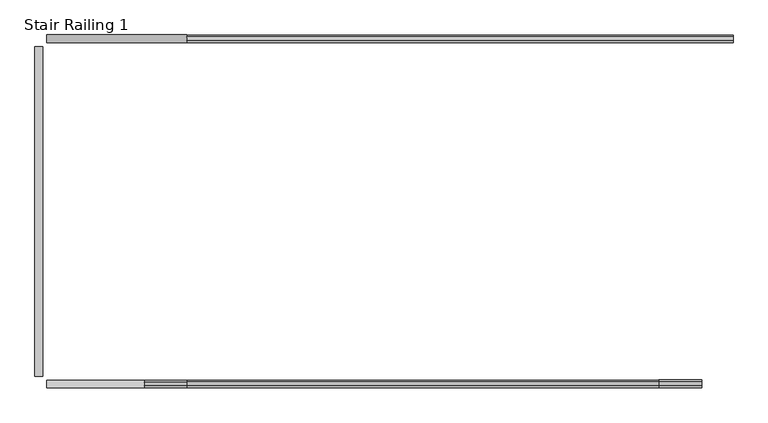
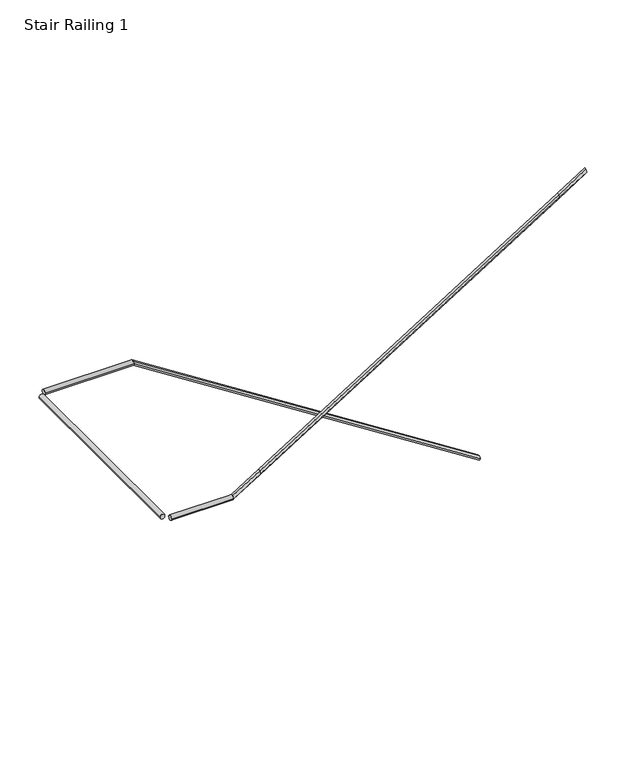
"""IFC4 building model written with IfcOpenShell, lengths in millimetres: railing geometry, Stair Railing 1."""

import ifcopenshell
import ifcopenshell.guid

model = None  # the IFC model being written
_history = None  # IfcOwnerHistory: only IFC2X3 demands one
_inside = {}  # id of a spatial element -> (the spatial element, [elements in it])
_under = {}  # id of a project, library or spatial element -> (it, [spatial elements below it])
_declared = {}  # id of a project -> (the project, [libraries it declares])
_typed = {}  # id of a type object -> (the type object, [elements of that type])
_made_of = {}  # id of a material, layer set ... -> (it, [elements and type objects made of it])


def new_model(schema):
    """Start an empty IFC model of exactly this schema.

    Asked for "IFC4X3", IfcOpenShell would pick the latest addendum, in which some entities
    have other attributes; the version numbers below select the first issue.
    IFC2X3 requires an IfcOwnerHistory on every rooted entity: one is made here for all.
    """
    global model, _history
    if schema == "IFC4X3":
        model = ifcopenshell.file(schema_version=(4, 3, 0, 0))
    else:
        model = ifcopenshell.file(schema=schema)
    _inside.clear()
    _under.clear()
    _declared.clear()
    _typed.clear()
    _made_of.clear()
    _history = None
    if model.schema == "IFC2X3":
        org = make("IfcOrganization", Name="unknown")
        user = make(
            "IfcPersonAndOrganization",
            ThePerson=make("IfcPerson", FamilyName="unknown"),
            TheOrganization=org,
        )
        app = make(
            "IfcApplication",
            ApplicationDeveloper=org,
            Version="unknown",
            ApplicationFullName="unknown",
            ApplicationIdentifier="unknown",
        )
        _history = make(
            "IfcOwnerHistory",
            OwningUser=user,
            OwningApplication=app,
            ChangeAction="ADDED",
            CreationDate=0,
        )
    return model


def make(cls, **values):
    """One entity of the class cls with the attributes given. An attribute that is None is left unset."""
    return model.create_entity(
        cls, **{name: value for name, value in values.items() if value is not None}
    )


def rooted(cls, **values):
    """An entity with a GlobalId (a new one), such as an element, a storey or a relation."""
    return make(cls, GlobalId=ifcopenshell.guid.new(), OwnerHistory=_history, **values)


def si_unit(unit_type, name, prefix=None):
    """IfcSIUnit, for example si_unit("LENGTHUNIT", "METRE", prefix="MILLI")."""
    return make("IfcSIUnit", UnitType=unit_type, Prefix=prefix, Name=name)


def assignment(units):
    """IfcUnitAssignment: the units of a project."""
    return None if units is None else make("IfcUnitAssignment", Units=units)


def point(xyz):
    """IfcCartesianPoint."""
    return None if xyz is None else make("IfcCartesianPoint", Coordinates=xyz)


def direction(xyz):
    """IfcDirection."""
    return None if xyz is None else make("IfcDirection", DirectionRatios=xyz)


def frame(location, z_axis=None, x_axis=None):
    """IfcAxis2Placement3D, a coordinate frame: its origin and axes. An axis left out is left unset."""
    return make(
        "IfcAxis2Placement3D",
        Location=point(location),
        Axis=direction(z_axis),
        RefDirection=direction(x_axis),
    )


def origin():
    """The frame at (0, 0, 0) with its axes left unset."""
    return frame((0.0, 0.0, 0.0))


def place(relative_to, where):
    """IfcLocalPlacement: puts the frame where relative to a parent placement (None: the world)."""
    return make(
        "IfcLocalPlacement", PlacementRelTo=relative_to, RelativePlacement=where
    )


def context(
    kind, dimensions, precision=None, world=None, true_north=None, identifier=None
):
    """IfcGeometricRepresentationContext, for example the 3D "Model" context."""
    return make(
        "IfcGeometricRepresentationContext",
        ContextIdentifier=identifier,
        ContextType=kind,
        CoordinateSpaceDimension=dimensions,
        Precision=precision,
        WorldCoordinateSystem=world,
        TrueNorth=true_north,
    )


def project(units=None, contexts=None):
    """IfcProject with its units and contexts."""
    return rooted(
        "IfcProject",
        Name="project",
        RepresentationContexts=contexts,
        UnitsInContext=assignment(units),
    )


def spatial(cls, under=None, at=None, **own):
    """A site, building, storey or space (cls), placed at a placement, below another one or the project."""
    s = rooted(cls, ObjectPlacement=at, **own)
    if under is not None:
        _under.setdefault(under.id(), (under, []))[1].append(s)
    return s


def circle_curve(where, radius):
    """IfcCircle in the frame where."""
    return make("IfcCircle", Position=where, Radius=radius)


def faces_of(points, faces, orient=None, outer=None):
    """IfcFace entities. A face is a list of loops; a loop is a list of indices into points, from 0.

    orient and outer hold one flag for each loop. By default every Orientation is true, the
    first loop of a face is its IfcFaceOuterBound and the others are IfcFaceBound.
    """
    made = []
    for i, loops in enumerate(faces):
        bounds = []
        for j, loop in enumerate(loops):
            is_outer = j == 0 if outer is None else outer[i][j]
            bounds.append(
                make(
                    "IfcFaceOuterBound" if is_outer else "IfcFaceBound",
                    Bound=make("IfcPolyLoop", Polygon=[points[k] for k in loop]),
                    Orientation=True if orient is None else orient[i][j],
                )
            )
        made.append(make("IfcFace", Bounds=bounds))
    return made


def faceted_brep(points, faces, orient=None, outer=None, voids=None):
    """IfcFacetedBrep: a solid bounded by flat faces; with voids (closed shells), ...WithVoids."""
    shared = [point(p) for p in points]
    hull = make("IfcClosedShell", CfsFaces=faces_of(shared, faces, orient, outer))
    if voids is None:
        return make("IfcFacetedBrep", Outer=hull)
    return make(
        "IfcFacetedBrepWithVoids",
        Outer=hull,
        Voids=[
            make(cls, CfsFaces=faces_of(shared, fs, o, b)) for cls, fs, o, b in voids
        ],
    )


def shape(context_of_items, identifier, shape_type, items):
    """IfcShapeRepresentation: the items that make up one representation, for example the "Body"."""
    return make(
        "IfcShapeRepresentation",
        ContextOfItems=context_of_items,
        RepresentationIdentifier=identifier,
        RepresentationType=shape_type,
        Items=items,
    )


def source(mapping_origin, context_of_items, identifier, shape_type, items):
    """IfcRepresentationMap: a shape defined once, which mapped items show again and again."""
    return make(
        "IfcRepresentationMap",
        MappingOrigin=mapping_origin,
        MappedRepresentation=shape(context_of_items, identifier, shape_type, items),
    )


def transform(
    local_origin,
    x_axis=None,
    y_axis=None,
    z_axis=None,
    scale=None,
    scale2=None,
    scale3=None,
    uniform=True,
):
    """IfcCartesianTransformationOperator3D, or its non-uniform kind. x_axis, y_axis, z_axis: its Axis1, 2, 3."""
    if uniform:
        return make(
            "IfcCartesianTransformationOperator3D",
            Axis1=direction(x_axis),
            Axis2=direction(y_axis),
            LocalOrigin=point(local_origin),
            Scale=scale,
            Axis3=direction(z_axis),
        )
    return make(
        "IfcCartesianTransformationOperator3DnonUniform",
        Axis1=direction(x_axis),
        Axis2=direction(y_axis),
        LocalOrigin=point(local_origin),
        Scale=scale,
        Axis3=direction(z_axis),
        Scale2=scale2,
        Scale3=scale3,
    )


def mapped(mapping_source, mapping_target):
    """IfcMappedItem: shows the shape of a source again, moved by a transform."""
    return make(
        "IfcMappedItem", MappingSource=mapping_source, MappingTarget=mapping_target
    )


def made_of(thing, what):
    """Note that an element or type object is made of a material, layer set ...; save() writes the relation."""
    if what is not None:
        _made_of.setdefault(what.id(), (what, []))[1].append(thing)
    return thing


def element(
    cls,
    number,
    at=None,
    inside=None,
    cuts=None,
    type_object=None,
    material=None,
    context=None,
    identifier="Body",
    shape_type=None,
    held_by="IfcProductDefinitionShape",
    body=None,
    shapes=None,
    **own,
):
    """One element of the class cls, such as IfcWall. Its Tag is "e" and its number.

    at: its placement. inside: the storey or other place that contains it. cuts: it is an
    opening in that element (IfcRelVoidsElement). A single representation is given by context,
    identifier, shape_type and body (its items); several are given by shapes. held_by: the class
    of the entity that holds the representations. save() writes the other relations.
    """
    e = rooted(cls, Tag="e%d" % number, ObjectPlacement=at, **own)
    if body is not None:
        shapes = [shape(context, identifier, shape_type, body)]
    if shapes is not None:
        e.Representation = make(held_by, Representations=shapes)
    if inside is not None:
        _inside.setdefault(inside.id(), (inside, []))[1].append(e)
    if cuts is not None:
        rooted(
            "IfcRelVoidsElement", RelatingBuildingElement=cuts, RelatedOpeningElement=e
        )
    if type_object is not None:
        _typed.setdefault(type_object.id(), (type_object, []))[1].append(e)
    return made_of(e, material)


def aggregate(whole, parts):
    """IfcRelAggregates: a whole, such as a stair, and the parts it consists of."""
    return rooted("IfcRelAggregates", RelatingObject=whole, RelatedObjects=parts)


def save(model, path):
    """Write the relations noted so far, then the file.

    IfcRelAggregates (storeys below a building ...), IfcRelContainedInSpatialStructure (elements
    in a storey), IfcRelDefinesByType, IfcRelAssociatesMaterial and IfcRelDeclares: one each for
    every whole, place, type object, material and project.
    """
    for whole, parts in _under.values():
        aggregate(whole, parts)
    for where, things in _inside.values():
        rooted(
            "IfcRelContainedInSpatialStructure",
            RelatedElements=things,
            RelatingStructure=where,
        )
    for kind, things in _typed.values():
        rooted("IfcRelDefinesByType", RelatedObjects=things, RelatingType=kind)
    for what, things in _made_of.values():
        rooted("IfcRelAssociatesMaterial", RelatedObjects=things, RelatingMaterial=what)
    for by, libraries in _declared.values():
        rooted("IfcRelDeclares", RelatingContext=by, RelatedDefinitions=libraries)
    model.write(path)


def plane_surface(at):
    """IfcPlane: the flat surface through the origin of the frame at, square to its z axis."""
    return make("IfcPlane", Position=at)


def cylinder_surface(at, radius):
    """IfcCylindricalSurface: all points at the distance radius from the z axis of the frame at."""
    return make("IfcCylindricalSurface", Position=at, Radius=radius)


def advanced_brep(points, edges, surfaces, faces):
    """IfcAdvancedBrep: a solid bounded by faces that lie on surfaces and meet in shared edges.

    An edge is (start, end): straight between two places in points (the first is 0);
    or (start, end, curve); or (start, end, curve, False) where it runs against its curve.
    A face is (place in surfaces, loops), or (place, loops, False) where it looks against
    its surface's normal. A loop lists edges by number (the first is 1), with a minus sign
    where the edge is run from its end to its start. The first loop is the outer one.
    """
    corners = [point(p) for p in points]
    vertices = [make("IfcVertexPoint", VertexGeometry=c) for c in corners]
    made = []
    for start, end, *more in edges:
        made.append(
            make(
                "IfcEdgeCurve",
                EdgeStart=vertices[start],
                EdgeEnd=vertices[end],
                EdgeGeometry=more[0] if more else make("IfcPolyline", Points=[corners[start], corners[end]]),
                SameSense=more[1] if len(more) > 1 else True,
            )
        )
    hull = []
    for where, loops, *sense in faces:
        bounds = []
        for j, loop in enumerate(loops):
            ring = [make("IfcOrientedEdge", EdgeElement=made[abs(k) - 1], Orientation=k > 0) for k in loop]
            bounds.append(
                make(
                    "IfcFaceOuterBound" if j == 0 else "IfcFaceBound",
                    Bound=make("IfcEdgeLoop", EdgeList=ring),
                    Orientation=True,
                )
            )
        hull.append(make("IfcAdvancedFace", Bounds=bounds, FaceSurface=surfaces[where], SameSense=sense[0] if sense else True))
    return make("IfcAdvancedBrep", Outer=make("IfcClosedShell", CfsFaces=hull))


def stair_railing_1_d57b5f3b(model_context):
    return source(origin(), model_context, "Body", "SolidModel", [
        faceted_brep([(46975.6613811, 47258.2865351, 13752.6888889), (46975.6613811, 47245.5865351, 13730.6918436), (46975.6613811, 47220.1865351, 13730.6918436), (46975.6613811, 47207.4865351, 13752.6888889), (46975.6613811, 47220.1865351, 13774.6859341), (46975.6613811, 47245.5865351, 13774.6859341), (50534.1355635, 47258.2865351, 11477.9777778), (50534.1355635, 47245.5865351, 11499.974823), (50534.1355635, 47220.1865351, 11499.974823), (50534.1355635, 47207.4865351, 11477.9777778), (50534.1355635, 47220.1865351, 11455.9807325), (50534.1355635, 47245.5865351, 11455.9807325)], [[[0, 1, 2, 3, 4, 5]], [[6, 7, 8, 9, 10, 11]], [[1, 0, 6, 11]], [[2, 1, 11, 10]], [[3, 2, 10, 9]], [[4, 3, 9, 8]], [[5, 4, 8, 7]], [[0, 5, 7, 6]]]),
        advanced_brep(
        [(46061.2613811, 47258.2865351, 13752.6888889), (46061.2613811, 47207.4865351, 13752.6888889), (46975.6613811, 47258.2865351, 13752.6888889), (46975.6613811, 47207.4865351, 13752.6888889)],
        [
            (0, 1, circle_curve(frame((46061.2613811, 47232.8865351, 13752.6888889), z_axis=(-1.0, 0.0, 0.0), x_axis=(0.0, 1.0, 0.0)), 25.4)),
            (1, 0, circle_curve(frame((46061.2613811, 47232.8865351, 13752.6888889), z_axis=(-1.0, 0.0, 0.0), x_axis=(0.0, 1.0, 0.0)), 25.4)),
            (2, 3, circle_curve(frame((46975.6613811, 47232.8865351, 13752.6888889), z_axis=(1.0, 0.0, 0.0), x_axis=(0.0, 1.0, 0.0)), 25.4)),
            (3, 2, circle_curve(frame((46975.6613811, 47232.8865351, 13752.6888889), z_axis=(1.0, 0.0, 0.0), x_axis=(0.0, 1.0, 0.0)), 25.4)),
            (0, 2),
            (3, 1),
        ],
        [
            plane_surface(frame((46061.2613811, 47258.2865351, 13727.2888889), z_axis=(-1.0, 0.0, 0.0), x_axis=(0.0, -1.0, 0.0))),
            plane_surface(frame((46975.6613811, 47258.2865351, 13727.2888889), z_axis=(1.0, 0.0, 0.0), x_axis=(0.0, 1.0, 0.0))),
            cylinder_surface(frame((46975.6613811, 47232.8865351, 13752.6888889), z_axis=(-1.0, 0.0, 0.0), x_axis=(0.0, 1.0, 0.0)), 25.4),
        ],
        [
            (0, [[1, 2]]),
            (1, [[3, 4]]),
            (2, [[-1, 5, -4, 6]]),
            (2, [[-2, -6, -3, -5]]),
        ],
    ),
        advanced_brep(
        [(45985.0613811, 45032.0030566, 13752.6888889), (46035.8613811, 45032.0030566, 13752.6888889), (45985.0613811, 47182.0865351, 13752.6888889), (46035.8613811, 47182.0865351, 13752.6888889)],
        [
            (0, 1, circle_curve(frame((46010.4613811, 45032.0030566, 13752.6888889), z_axis=(0.0, -1.0, 0.0), x_axis=(-1.0, 0.0, 0.0)), 25.4)),
            (1, 0, circle_curve(frame((46010.4613811, 45032.0030566, 13752.6888889), z_axis=(0.0, -1.0, 0.0), x_axis=(-1.0, 0.0, 0.0)), 25.4)),
            (2, 3, circle_curve(frame((46010.4613811, 47182.0865351, 13752.6888889), z_axis=(0.0, 1.0, 0.0), x_axis=(-1.0, 0.0, 0.0)), 25.4)),
            (3, 2, circle_curve(frame((46010.4613811, 47182.0865351, 13752.6888889), z_axis=(0.0, 1.0, 0.0), x_axis=(-1.0, 0.0, 0.0)), 25.4)),
            (0, 2),
            (3, 1),
        ],
        [
            plane_surface(frame((45985.0613811, 45032.0030566, 13727.2888889), z_axis=(0.0, -1.0, 0.0), x_axis=(0.0, 0.0, -1.0))),
            plane_surface(frame((45985.0613811, 47182.0865351, 13727.2888889), z_axis=(0.0, 1.0, 0.0), x_axis=(0.0, 0.0, 1.0))),
            cylinder_surface(frame((46010.4613811, 47182.0865351, 13752.6888889), z_axis=(0.0, -1.0, 0.0), x_axis=(-1.0, 0.0, 0.0)), 25.4),
        ],
        [
            (0, [[1, 2]]),
            (1, [[3, 4]]),
            (2, [[-1, 5, -4, 6]]),
            (2, [[-2, -6, -3, -5]]),
        ],
    ),
        advanced_brep(
        [(46696.2613811, 44955.8030566, 13752.6888889), (46696.2613811, 45006.6030566, 13752.6888889), (46061.2613811, 44955.8030566, 13752.6888889), (46061.2613811, 45006.6030566, 13752.6888889)],
        [
            (0, 1, circle_curve(frame((46696.2613811, 44981.2030566, 13752.6888889), z_axis=(1.0, 0.0, 0.0), x_axis=(0.0, -1.0, 0.0)), 25.4)),
            (1, 0, circle_curve(frame((46696.2613811, 44981.2030566, 13752.6888889), z_axis=(1.0, 0.0, 0.0), x_axis=(0.0, -1.0, 0.0)), 25.4)),
            (2, 3, circle_curve(frame((46061.2613811, 44981.2030566, 13752.6888889), z_axis=(-1.0, 0.0, 0.0), x_axis=(0.0, -1.0, 0.0)), 25.4)),
            (3, 2, circle_curve(frame((46061.2613811, 44981.2030566, 13752.6888889), z_axis=(-1.0, 0.0, 0.0), x_axis=(0.0, -1.0, 0.0)), 25.4)),
            (0, 2),
            (3, 1),
        ],
        [
            plane_surface(frame((46696.2613811, 44955.8030566, 13727.2888889), z_axis=(1.0, 0.0, 0.0), x_axis=(0.0, 1.0, 0.0))),
            plane_surface(frame((46061.2613811, 44955.8030566, 13727.2888889), z_axis=(-1.0, 0.0, 0.0), x_axis=(0.0, -1.0, 0.0))),
            cylinder_surface(frame((46061.2613811, 44981.2030566, 13752.6888889), z_axis=(1.0, 0.0, 0.0), x_axis=(0.0, -1.0, 0.0)), 25.4),
        ],
        [
            (0, [[1, 2]]),
            (1, [[3, 4]]),
            (2, [[-1, 5, -4, 6]]),
            (2, [[-2, -6, -3, -5]]),
        ],
    ),
        faceted_brep([(46975.6613811, 44955.8030566, 13927.6666667), (46975.6613811, 44968.5030566, 13905.6696214), (46975.6613811, 44993.9030566, 13905.6696214), (46975.6613811, 45006.6030566, 13927.6666667), (46975.6613811, 44993.9030566, 13949.6637119), (46975.6613811, 44968.5030566, 13949.6637119), (46696.2613811, 44955.8030566, 13752.6888889), (46696.2613811, 44968.5030566, 13774.6859341), (46696.2613811, 44993.9030566, 13774.6859341), (46696.2613811, 45006.6030566, 13752.6888889), (46696.2613811, 44993.9030566, 13730.6918436), (46696.2613811, 44968.5030566, 13730.6918436)], [[[0, 1, 2, 3, 4, 5]], [[6, 7, 8, 9, 10, 11]], [[1, 0, 6, 11]], [[2, 1, 11, 10]], [[3, 2, 10, 9]], [[4, 3, 9, 8]], [[5, 4, 8, 7]], [[0, 5, 7, 6]]]),
        faceted_brep([(50049.0613811, 44955.8030566, 15852.4222222), (50049.0613811, 44968.5030566, 15830.425177), (50049.0613811, 44993.9030566, 15830.425177), (50049.0613811, 45006.6030566, 15852.4222222), (50049.0613811, 44993.9030566, 15874.4192675), (50049.0613811, 44968.5030566, 15874.4192675), (46975.6613811, 44955.8030566, 13927.6666667), (46975.6613811, 44968.5030566, 13949.6637119), (46975.6613811, 44993.9030566, 13949.6637119), (46975.6613811, 45006.6030566, 13927.6666667), (46975.6613811, 44993.9030566, 13905.6696214), (46975.6613811, 44968.5030566, 13905.6696214)], [[[0, 1, 2, 3, 4, 5]], [[6, 7, 8, 9, 10, 11]], [[1, 0, 6, 11]], [[2, 1, 11, 10]], [[3, 2, 10, 9]], [[4, 3, 9, 8]], [[5, 4, 8, 7]], [[0, 5, 7, 6]]]),
        faceted_brep([(50328.4613811, 44955.8030566, 16027.4), (50328.4613811, 44968.5030566, 16005.4029547), (50328.4613811, 44993.9030566, 16005.4029547), (50328.4613811, 45006.6030566, 16027.4), (50328.4613811, 44993.9030566, 16049.3970453), (50328.4613811, 44968.5030566, 16049.3970453), (50049.0613811, 44955.8030566, 15852.4222222), (50049.0613811, 44968.5030566, 15874.4192675), (50049.0613811, 44993.9030566, 15874.4192675), (50049.0613811, 45006.6030566, 15852.4222222), (50049.0613811, 44993.9030566, 15830.425177), (50049.0613811, 44968.5030566, 15830.425177)], [[[0, 1, 2, 3, 4, 5]], [[6, 7, 8, 9, 10, 11]], [[1, 0, 6, 11]], [[2, 1, 11, 10]], [[3, 2, 10, 9]], [[4, 3, 9, 8]], [[5, 4, 8, 7]], [[0, 5, 7, 6]]]),
    ])


if __name__ == "__main__":
    model = new_model("IFC4")
    model_context = context("Model", 3, world=origin())
    ifc_project = project(units=[si_unit("LENGTHUNIT", "METRE", prefix="MILLI")], contexts=[model_context])
    site = spatial("IfcSite", under=ifc_project)
    building = spatial("IfcBuilding", under=site)
    placement = place(None, origin())
    stair_railing_1_shape = stair_railing_1_d57b5f3b(model_context)
    element("IfcRailing", 1, ObjectType="Stair Railing 1", at=placement, inside=building, context=model_context, shape_type="MappedRepresentation", body=[
        mapped(stair_railing_1_shape, transform((0.0, 0.0, 0.0), x_axis=(1.0, 0.0, 0.0), y_axis=(0.0, 1.0, 0.0), z_axis=(0.0, 0.0, 1.0))),
    ])
    save(model, "model.ifc")
